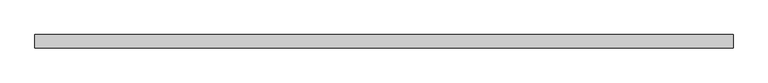
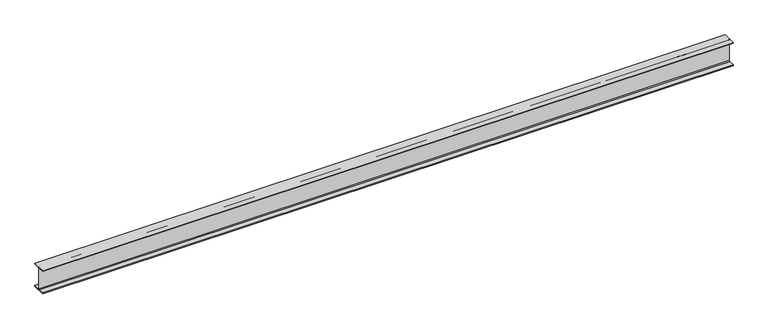
"""IFC4 building model written with IfcOpenShell, lengths in millimetres: beam geometry, Old_Steel Beam_H-KSD3502 : H_SB_ASB_H-300×300x10x15."""

from ifc_helpers import new_model, si_unit, point, frame, frame_2d, origin, place, context, project, spatial, polyline, circle_curve, trimmed, segment, composite_curve, outline, extrude, source, transform, mapped, element, save


def beam_f7cbd3fc(model_context):
    return source(origin(), model_context, "Body", "SweptSolid", [
        extrude(outline(composite_curve([segment(polyline([(82.5, -141.5), (82.5, -151.7), (-82.5, -151.7), (-82.5, -141.5), (-11.9, -141.5)]), True, "CONTINUOUS"), segment(trimmed(circle_curve(frame_2d((-11.9, -132.6)), 8.9), [point((-11.9, -141.5))], [point((-3.0, -132.6))], True, "CARTESIAN"), True, "CONTINUOUS"), segment(polyline([(-3.0, -132.6), (-3.0, 132.6)]), True, "CONTINUOUS"), segment(trimmed(circle_curve(frame_2d((-11.9, 132.6)), 8.9), [point((-3.0, 132.6))], [point((-11.9, 141.5))], True, "CARTESIAN"), True, "CONTINUOUS"), segment(polyline([(-11.9, 141.5), (-82.5, 141.5), (-82.5, 151.7), (82.5, 151.7), (82.5, 141.5), (11.9, 141.5)]), True, "CONTINUOUS"), segment(trimmed(circle_curve(frame_2d((11.9, 132.6)), 8.9), [point((11.9, 141.5))], [point((3.0, 132.6))], True, "CARTESIAN"), True, "CONTINUOUS"), segment(polyline([(3.0, 132.6), (3.0, -132.6)]), True, "CONTINUOUS"), segment(trimmed(circle_curve(frame_2d((11.9, -132.6)), 8.9), [point((3.0, -132.6))], [point((11.9, -141.5))], True, "CARTESIAN"), True, "CONTINUOUS"), segment(polyline([(11.9, -141.5), (82.5, -141.5)]), True, "CONTINUOUS")], self_intersect=False)), frame((-4331.4958952, 0.0, 0.0), z_axis=(1.0, 0.0, 0.0), x_axis=(0.0, 1.0, 0.0)), (0.0, 0.0, 1.0), 8594.5528849),
    ])


if __name__ == "__main__":
    model = new_model("IFC4")
    model_context = context("Model", 3, world=origin())
    ifc_project = project(units=[si_unit("LENGTHUNIT", "METRE", prefix="MILLI")], contexts=[model_context])
    site = spatial("IfcSite", under=ifc_project)
    building = spatial("IfcBuilding", under=site)
    placement = place(None, origin())
    beam_shape = beam_f7cbd3fc(model_context)
    element("IfcBeam", 1, ObjectType="Old_Steel Beam_H-KSD3502 : H_SB_ASB_H-300×300x10x15", at=placement, inside=building, context=model_context, shape_type="MappedRepresentation", body=[
        mapped(beam_shape, transform((0.0, 0.0, 0.0), x_axis=(1.0, 0.0, 0.0), y_axis=(0.0, 1.0, 0.0), z_axis=(0.0, 0.0, 1.0))),
    ])
    save(model, "model.ifc")

# Revit data of these elements
# Type "Old_Steel Beam_H-KSD3502 : H_SB_ASB_H-300×300x10x15"
#   Width = 30.0 cm
#   Web Thickness = 1.0 cm
#   Web Fillet = 1.8 cm
#   Warping Constant = 1370670.0 cm⁶
#   Torsional Moment of Inertia = 77.00 cm⁴
#   Torsional Modulus = 1.0 cm³
#   Section Area = 119.8 cm²
#   Plastic Modulus weak axis = 684.0 cm³
#   Plastic Modulus strong axis = 1500.0 cm³
#   Perimeter = 1.75 m²/m
#   Nominal Weight = 94.00 kgf/m
#   Moment of Inertia weak axis = 6750.00 cm⁴
#   Moment of Inertia strong axis = 20400.00 cm⁴
#   Height = 30.0 cm
#   Flange Thickness = 1.5 cm
#   Elastic Modulus weak axis = 450.0 cm³
#   Elastic Modulus strong axis = 1360.0 cm³
#   Centroid Vertical = 15.0 cm
#   Centroid Horizontal = 15.0 cm
#   Length [instance default] = 1.5240 m
#   Structural Material [instance default] = Steel, 45-345
#   Assembly Code = ""
# Element 1 (IfcBeam, "Old_Steel Beam_H-KSD3502 : H_SB_ASB_H-300×300x10x15")
#   Structural Material = none
# Materials
#   "Steel, 45-345": class "Metal", colour RGB 189 187 185, transparency 0, Description = "Steel 345 MPa", Cost = 0
